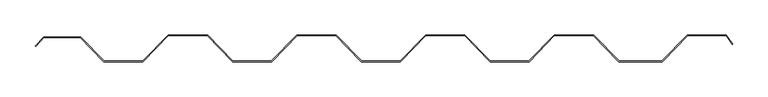
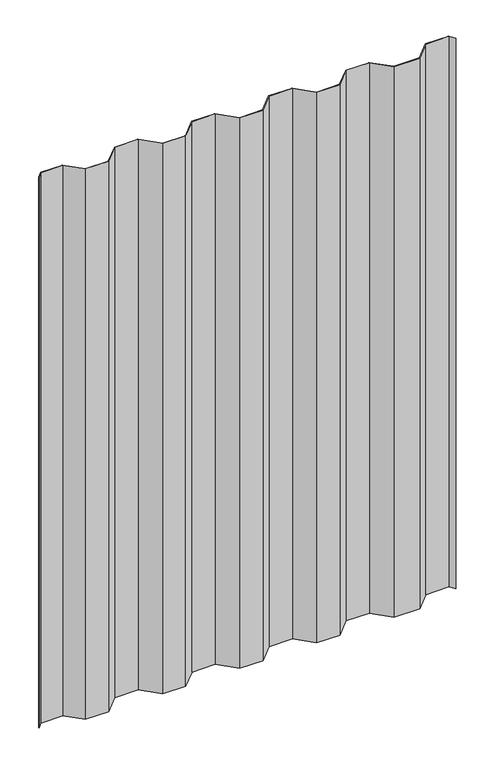
"""IFC4 building model written with IfcOpenShell, lengths in millimetres: proxy geometry, Generic Models 2:Generic Models 2:310765:Generic Models 2:310765 : Generic Models 2:Generic Models 2:310765:282 : Generic Models 2:Generic Models 2:310765:Generic Models 2:310765 : Generic Models 2:Generic Models 2:310765:300385."""

from ifc_helpers import new_model, si_unit, frame, origin, place, context, project, spatial, polyline, outline, extrude, source, transform, mapped, element, save


def generic_models_27c1aacb(model_context):
    return source(origin(), model_context, "Body", "SweptSolid", [
        extrude(outline(polyline([(793296.6908851, -578743.0895469), (793349.2846908, -578743.0895469), (793382.9166755, -578777.6476341), (793437.4250755, -578777.6476341), (793473.5872672, -578740.3413841), (793529.6344839, -578740.3413841), (793565.7966755, -578777.6476341), (793620.3050755, -578777.6476341), (793656.4672672, -578740.3413841), (793712.5144839, -578740.3413841), (793748.6766755, -578777.6476341), (793803.1850755, -578777.6476341), (793839.3472672, -578740.3413841), (793895.3944839, -578740.3413841), (793931.5566755, -578777.6476341), (793986.0650755, -578777.6476341), (794022.2272672, -578740.3413841), (794078.2744839, -578740.3413841), (794114.4366755, -578777.6476341), (794175.2950755, -578777.6476341), (794211.4572672, -578740.3413841), (794266.7350755, -578740.3413841), (794275.9134457, -578753.4494551), (794275.2632437, -578753.9047314), (794266.3218754, -578741.1351341), (794211.7933127, -578741.1351341), (794175.6311211, -578778.4413841), (794114.10063, -578778.4413841), (794077.9384383, -578741.1351341), (794022.5633127, -578741.1351341), (793986.4011211, -578778.4413841), (793931.22063, -578778.4413841), (793895.0584383, -578741.1351341), (793839.6833127, -578741.1351341), (793803.5211211, -578778.4413841), (793748.34063, -578778.4413841), (793712.1784383, -578741.1351341), (793656.8033127, -578741.1351341), (793620.6411211, -578778.4413841), (793565.46063, -578778.4413841), (793529.2984383, -578741.1351341), (793473.9233127, -578741.1351341), (793437.7611211, -578778.4413841), (793382.5815612, -578778.4413841), (793348.9495764, -578743.8832969), (793297.0432224, -578743.8832969), (793285.3971106, -578756.7595897), (793284.8351388, -578756.1976179), (793296.6908851, -578743.0895469)])), frame((0.0, 0.0, 4786.4066729), z_axis=(0.0, 0.0, 1.0), x_axis=(1.0, 0.0, 0.0)), (0.0, 0.0, 1.0), 1379.4433271),
    ])


if __name__ == "__main__":
    model = new_model("IFC4")
    model_context = context("Model", 3, world=origin())
    ifc_project = project(units=[si_unit("LENGTHUNIT", "METRE", prefix="MILLI")], contexts=[model_context])
    site = spatial("IfcSite", under=ifc_project)
    building = spatial("IfcBuilding", under=site)
    placement = place(None, origin())
    generic_models_shape = generic_models_27c1aacb(model_context)
    element("IfcBuildingElementProxy", 1, Name="Generic Models 2:Generic Models 2:310765:Generic Models 2:310765 : Generic Models 2:Generic Models 2:310765:282 : Generic Models 2:Generic Models 2:310765:Generic Models 2:310765 : Generic Models 2:Generic Models 2:310765:300385", ObjectType="Generic Models 2:Generic Models 2:310765:Generic Models 2:310765 : Generic Models 2:Generic Models 2:310765:282 : Generic Models 2:Generic Models 2:310765:Generic Models 2:310765 : Generic Models 2:Generic Models 2:310765:300385", at=placement, inside=building, context=model_context, shape_type="MappedRepresentation", body=[
        mapped(generic_models_shape, transform((0.0, 0.0, 0.0), x_axis=(1.0, 0.0, 0.0), y_axis=(0.0, 1.0, 0.0), z_axis=(0.0, 0.0, 1.0))),
    ])
    save(model, "model.ifc")

# Revit data of these elements
# Type "Generic Models 2:Generic Models 2:310765:Generic Models 2:310765 : Generic Models 2:Generic Models 2:310765:282 : Generic Models 2:Generic Models 2:310765:Generic Models 2:310765 : Generic Models 2:Generic Models 2:310765:300385"
#   NameOverride = "Generic Models 2:Generic Models 2:310765:Generic Models 2:310765 : Generic Models 2:Generic Models 2:310765:300385"
#   ObjectTypeOverride = "Generic Models 2:310765 : Generic Models 2:Generic Models 2:310765"
#   Reference = "Generic Models 2"
#   Tag = "300385"
# Element 1 (IfcBuildingElementProxy, "Generic Models 2:Generic Models 2:310765:Generic Models 2:310765 : Generic Models 2:Generic Models 2:310765:282 : Generic Models 2:Generic Models 2:310765:Generic Models 2:310765 : Generic Models 2:Generic Models 2:310765:300385")
#   Materials on its faces: "VERTICAL CORRUGATED METAL PANEL - EXPOSED FASTENERS - (MBCI 7.2 PANEL)"
# Materials
#   "VERTICAL CORRUGATED METAL PANEL - EXPOSED FASTENERS - (MBCI 7.2 PANEL)": class "Generic", colour RGB 120 120 120, transparency 0, Cost = 0
